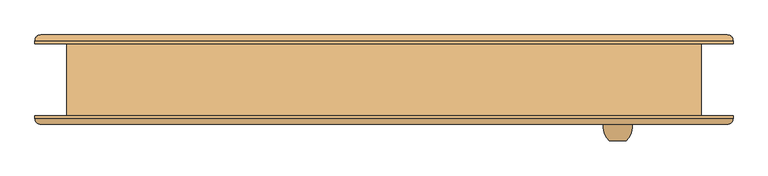
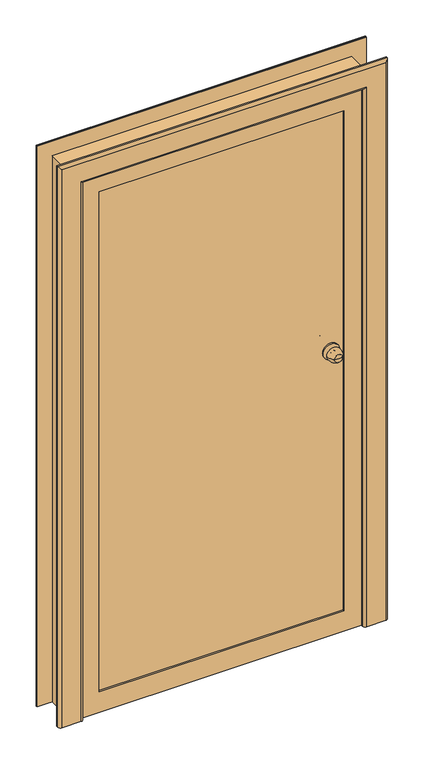
"""IFC4 building model written with IfcOpenShell, lengths in millimetres: door geometry, Наружная дверь 1-Навесная - Один проем наружу с порогом - 31173-2003 : ДСН КЛН  М1 УЗ 2100-1100 ГОСТ 31173-2003."""

from ifc_helpers import new_model, si_unit, point, frame, origin, place, context, project, spatial, polyline, circle_curve, ellipse_curve, trimmed, outline, extrude, faceted_brep, source, transform, mapped, element, save
from ifc_brep_helpers import plane_surface, cylinder_surface, revolved_surface, advanced_brep


def door_7e4ce2f0(model_context):
    return source(origin(), model_context, "Body", "SolidModel", [
        advanced_brep(
        [(390.0, -105.5, 1100.0), (405.0, -105.5, 1100.0), (420.0, -105.5, 1100.0), (430.0, -75.5, 1100.0), (380.0, -75.5, 1100.0), (423.0, -75.5, 1100.0), (387.0, -75.5, 1100.0), (415.0, -67.5, 1100.0), (395.0, -67.5, 1100.0), (415.0, -61.5, 1100.0), (395.0, -61.5, 1100.0), (435.0, -61.5, 1100.0), (375.0, -61.5, 1100.0), (435.0, -55.5, 1100.0), (375.0, -55.5, 1100.0)],
        [
            (0, 1),
            (1, 2),
            (2, 0, circle_curve(frame((405.0, -105.5, 1100.0), z_axis=(0.0, -1.0, 0.0), x_axis=(1.0, 0.0, 0.0)), 15.0)),
            (0, 2, circle_curve(frame((405.0, -105.5, 1100.0), z_axis=(0.0, -1.0, 0.0), x_axis=(1.0, 0.0, 0.0)), 15.0)),
            (2, 3, circle_curve(frame((395.3773735, -80.6257912, 1100.0), z_axis=(0.0, 0.0, 1.0), x_axis=(-1.0, 0.0, 0.0)), 35.0)),
            (3, 4, circle_curve(frame((405.0, -75.5, 1100.0), z_axis=(0.0, -1.0, 0.0), x_axis=(1.0, 0.0, 0.0)), 25.0)),
            (4, 0, circle_curve(frame((414.6226265, -80.6257912, 1100.0), z_axis=(0.0, 0.0, 1.0), x_axis=(1.0, 0.0, 0.0)), 35.0)),
            (4, 3, circle_curve(frame((405.0, -75.5, 1100.0), z_axis=(0.0, -1.0, 0.0), x_axis=(1.0, 0.0, 0.0)), 25.0)),
            (3, 5),
            (5, 6, circle_curve(frame((405.0, -75.5, 1100.0), z_axis=(0.0, -1.0, 0.0), x_axis=(1.0, 0.0, 0.0)), 18.0)),
            (6, 4),
            (6, 5, circle_curve(frame((405.0, -75.5, 1100.0), z_axis=(0.0, -1.0, 0.0), x_axis=(1.0, 0.0, 0.0)), 18.0)),
            (5, 7, circle_curve(frame((423.0, -67.5, 1100.0), z_axis=(0.0, 0.0, -1.0), x_axis=(-1.0, 0.0, 0.0)), 8.0)),
            (7, 8, circle_curve(frame((405.0, -67.5, 1100.0), z_axis=(0.0, -1.0, 0.0), x_axis=(1.0, 0.0, 0.0)), 10.0)),
            (8, 6, circle_curve(frame((387.0, -67.5, 1100.0), z_axis=(0.0, 0.0, -1.0), x_axis=(1.0, 0.0, 0.0)), 8.0)),
            (8, 7, circle_curve(frame((405.0, -67.5, 1100.0), z_axis=(0.0, -1.0, 0.0), x_axis=(1.0, 0.0, 0.0)), 10.0)),
            (7, 9),
            (9, 10, circle_curve(frame((405.0, -61.5, 1100.0), z_axis=(0.0, -1.0, 0.0), x_axis=(1.0, 0.0, 0.0)), 10.0)),
            (10, 8),
            (10, 9, circle_curve(frame((405.0, -61.5, 1100.0), z_axis=(0.0, -1.0, 0.0), x_axis=(1.0, 0.0, 0.0)), 10.0)),
            (11, 12, circle_curve(frame((405.0, -61.5, 1100.0), z_axis=(0.0, -1.0, 0.0), x_axis=(-1.0, 0.0, 0.0)), 30.0)),
            (12, 11, circle_curve(frame((405.0, -61.5, 1100.0), z_axis=(0.0, -1.0, 0.0), x_axis=(-1.0, 0.0, 0.0)), 30.0)),
            (13, 14, circle_curve(frame((405.0, -55.5, 1100.0), z_axis=(0.0, 1.0, 0.0), x_axis=(-1.0, 0.0, 0.0)), 30.0)),
            (14, 13, circle_curve(frame((405.0, -55.5, 1100.0), z_axis=(0.0, 1.0, 0.0), x_axis=(-1.0, 0.0, 0.0)), 30.0)),
            (12, 14),
            (13, 11),
        ],
        [
            plane_surface(frame((405.0, -105.5, 1100.0), z_axis=(0.0, -1.0, 0.0), x_axis=(1.0, 0.0, 0.0))),
            revolved_surface(trimmed(ellipse_curve(frame((395.3773735, -80.6257912, 1100.0), z_axis=(0.0, 0.0, 1.0), x_axis=(-1.0, 0.0, 0.0)), 35.0, 35.0), [point((420.0, -105.5, 1100.0))], [point((430.0, -75.5, 1100.0))], True, "CARTESIAN"), (405.0, -135.5, 1100.0), (0.0, 1.0, 0.0)),
            plane_surface(frame((405.0, -75.5, 1100.0), z_axis=(0.0, 1.0, 0.0), x_axis=(1.0, 0.0, 0.0))),
            revolved_surface(trimmed(ellipse_curve(frame((423.0, -67.5, 1100.0), z_axis=(0.0, 0.0, -1.0), x_axis=(-1.0, 0.0, 0.0)), 8.0, 8.0), [point((423.0, -75.5, 1100.0))], [point((415.0, -67.5, 1100.0))], True, "CARTESIAN"), (405.0, -135.5, 1100.0), (0.0, 1.0, 0.0)),
            cylinder_surface(frame((405.0, -135.5, 1100.0), z_axis=(0.0, 1.0, 0.0), x_axis=(1.0, 0.0, 0.0)), 10.0),
            plane_surface(frame((375.0, -61.5, 1100.0), z_axis=(0.0, -1.0, 0.0), x_axis=(0.0, 0.0, 1.0))),
            plane_surface(frame((375.0, -55.5, 1100.0), z_axis=(0.0, 1.0, 0.0), x_axis=(0.0, 0.0, -1.0))),
            cylinder_surface(frame((405.0, -55.5, 1100.0), z_axis=(0.0, -1.0, 0.0), x_axis=(-1.0, 0.0, 0.0)), 30.0),
        ],
        [
            (0, [[1, 2, 3]]),
            (0, [[-1, 4, -2]]),
            (1, [[5, 6, 7, -3]]),
            (1, [[-7, 8, -5, -4]]),
            (2, [[9, 10, 11, -6]]),
            (2, [[-11, 12, -9, -8]]),
            (3, [[13, 14, 15, -10]]),
            (3, [[-15, 16, -13, -12]]),
            (4, [[17, 18, 19, -14]]),
            (4, [[-19, 20, -17, -16]]),
            (5, [[21, 22], [-20, -18]]),
            (6, [[23, 24]]),
            (7, [[25, -23, 26, -22]]),
            (7, [[-26, -24, -25, -21]]),
        ],
    ),
        advanced_brep(
        [(420.0, 64.5, 1100.0), (405.0, 64.5, 1100.0), (390.0, 64.5, 1100.0), (380.0, 34.5, 1100.0), (430.0, 34.5, 1100.0), (387.0, 34.5, 1100.0), (423.0, 34.5, 1100.0), (395.0, 26.5, 1100.0), (415.0, 26.5, 1100.0), (395.0, 20.5, 1100.0), (415.0, 20.5, 1100.0), (375.0, 20.5, 1100.0), (435.0, 20.5, 1100.0), (375.0, 14.5, 1100.0), (435.0, 14.5, 1100.0)],
        [
            (0, 1),
            (1, 2),
            (2, 0, circle_curve(frame((405.0, 64.5, 1100.0), z_axis=(0.0, 1.0, 0.0), x_axis=(-1.0, 0.0, 0.0)), 15.0)),
            (0, 2, circle_curve(frame((405.0, 64.5, 1100.0), z_axis=(0.0, 1.0, 0.0), x_axis=(-1.0, 0.0, 0.0)), 15.0)),
            (2, 3, circle_curve(frame((414.6226265, 39.6257912, 1100.0), z_axis=(0.0, 0.0, 1.0), x_axis=(1.0, 0.0, 0.0)), 35.0)),
            (3, 4, circle_curve(frame((405.0, 34.5, 1100.0), z_axis=(0.0, 1.0, 0.0), x_axis=(-1.0, 0.0, 0.0)), 25.0)),
            (4, 0, circle_curve(frame((395.3773735, 39.6257912, 1100.0), z_axis=(0.0, 0.0, 1.0), x_axis=(-1.0, 0.0, 0.0)), 35.0)),
            (4, 3, circle_curve(frame((405.0, 34.5, 1100.0), z_axis=(0.0, 1.0, 0.0), x_axis=(-1.0, 0.0, 0.0)), 25.0)),
            (3, 5),
            (5, 6, circle_curve(frame((405.0, 34.5, 1100.0), z_axis=(0.0, 1.0, 0.0), x_axis=(-1.0, 0.0, 0.0)), 18.0)),
            (6, 4),
            (6, 5, circle_curve(frame((405.0, 34.5, 1100.0), z_axis=(0.0, 1.0, 0.0), x_axis=(-1.0, 0.0, 0.0)), 18.0)),
            (5, 7, circle_curve(frame((387.0, 26.5, 1100.0), z_axis=(0.0, 0.0, -1.0), x_axis=(1.0, 0.0, 0.0)), 8.0)),
            (7, 8, circle_curve(frame((405.0, 26.5, 1100.0), z_axis=(0.0, 1.0, 0.0), x_axis=(-1.0, 0.0, 0.0)), 10.0)),
            (8, 6, circle_curve(frame((423.0, 26.5, 1100.0), z_axis=(0.0, 0.0, -1.0), x_axis=(-1.0, 0.0, 0.0)), 8.0)),
            (8, 7, circle_curve(frame((405.0, 26.5, 1100.0), z_axis=(0.0, 1.0, 0.0), x_axis=(-1.0, 0.0, 0.0)), 10.0)),
            (7, 9),
            (9, 10, circle_curve(frame((405.0, 20.5, 1100.0), z_axis=(0.0, 1.0, 0.0), x_axis=(-1.0, 0.0, 0.0)), 10.0)),
            (10, 8),
            (10, 9, circle_curve(frame((405.0, 20.5, 1100.0), z_axis=(0.0, 1.0, 0.0), x_axis=(-1.0, 0.0, 0.0)), 10.0)),
            (11, 12, circle_curve(frame((405.0, 20.5, 1100.0), z_axis=(0.0, 1.0, 0.0), x_axis=(1.0, 0.0, 0.0)), 30.0)),
            (12, 11, circle_curve(frame((405.0, 20.5, 1100.0), z_axis=(0.0, 1.0, 0.0), x_axis=(1.0, 0.0, 0.0)), 30.0)),
            (13, 14, circle_curve(frame((405.0, 14.5, 1100.0), z_axis=(0.0, -1.0, 0.0), x_axis=(1.0, 0.0, 0.0)), 30.0)),
            (14, 13, circle_curve(frame((405.0, 14.5, 1100.0), z_axis=(0.0, -1.0, 0.0), x_axis=(1.0, 0.0, 0.0)), 30.0)),
            (12, 14),
            (13, 11),
        ],
        [
            plane_surface(frame((405.0, 64.5, 1100.0), z_axis=(0.0, 1.0, 0.0), x_axis=(-1.0, 0.0, 0.0))),
            revolved_surface(trimmed(ellipse_curve(frame((414.6226265, 39.6257912, 1100.0), z_axis=(0.0, 0.0, 1.0), x_axis=(1.0, 0.0, 0.0)), 35.0, 35.0), [point((390.0, 64.5, 1100.0))], [point((380.0, 34.5, 1100.0))], True, "CARTESIAN"), (405.0, 94.5, 1100.0), (0.0, -1.0, 0.0)),
            plane_surface(frame((405.0, 34.5, 1100.0), z_axis=(0.0, -1.0, 0.0), x_axis=(-1.0, 0.0, 0.0))),
            revolved_surface(trimmed(ellipse_curve(frame((387.0, 26.5, 1100.0), z_axis=(0.0, 0.0, -1.0), x_axis=(1.0, 0.0, 0.0)), 8.0, 8.0), [point((387.0, 34.5, 1100.0))], [point((395.0, 26.5, 1100.0))], True, "CARTESIAN"), (405.0, 94.5, 1100.0), (0.0, -1.0, 0.0)),
            cylinder_surface(frame((405.0, 94.5, 1100.0), z_axis=(0.0, -1.0, 0.0), x_axis=(-1.0, 0.0, 0.0)), 10.0),
            plane_surface(frame((435.0, 20.5, 1100.0), z_axis=(0.0, 1.0, 0.0), x_axis=(0.0, 0.0, 1.0))),
            plane_surface(frame((435.0, 14.5, 1100.0), z_axis=(0.0, -1.0, 0.0), x_axis=(0.0, 0.0, -1.0))),
            cylinder_surface(frame((405.0, 14.5, 1100.0), z_axis=(0.0, 1.0, 0.0), x_axis=(1.0, 0.0, 0.0)), 30.0),
        ],
        [
            (0, [[1, 2, 3]]),
            (0, [[-1, 4, -2]]),
            (1, [[5, 6, 7, -3]]),
            (1, [[-7, 8, -5, -4]]),
            (2, [[9, 10, 11, -6]]),
            (2, [[-11, 12, -9, -8]]),
            (3, [[13, 14, 15, -10]]),
            (3, [[-15, 16, -13, -12]]),
            (4, [[17, 18, 19, -14]]),
            (4, [[-19, 20, -17, -16]]),
            (5, [[21, 22], [-20, -18]]),
            (6, [[23, 24]]),
            (7, [[25, -23, 26, -22]]),
            (7, [[-26, -24, -25, -21]]),
        ],
    ),
        faceted_brep([(485.0, 14.5, 42.0), (485.0, 9.5, 42.0), (-485.0, 9.5, 42.0), (-485.0, 14.5, 42.0), (485.0, 14.5, 2055.0), (485.0, 9.5, 2055.0), (-485.0, 9.5, 2055.0), (465.0, 9.5, 2035.0), (465.0, 9.5, 62.0), (-465.0, 9.5, 62.0), (-465.0, 9.5, 2035.0), (-485.0, 14.5, 2055.0), (465.0, -55.5, 2035.0), (465.0, -55.5, 62.0), (-465.0, -55.5, 62.0), (-465.0, -55.5, 2035.0)], [[[0, 1, 2, 3]], [[4, 5, 1, 0]], [[5, 6, 2, 1], [7, 8, 9, 10]], [[2, 6, 11, 3]], [[11, 4, 0, 3]], [[7, 12, 13, 8]], [[9, 8, 13, 14]], [[15, 10, 9, 14]], [[12, 15, 14, 13]], [[4, 11, 6, 5]], [[7, 10, 15, 12]]]),
        extrude(outline(polyline([(0.0, 515.0), (0.0, 530.0), (2100.0, 530.0), (2100.0, -530.0), (0.0, -530.0), (0.0, -515.0), (2085.0, -515.0), (2085.0, 515.0), (0.0, 515.0)])), frame((0.0, 7.5, 0.0), z_axis=(0.0, 1.0, 0.0), x_axis=(0.0, 0.0, 1.0)), (0.0, 0.0, 1.0), 55.0),
        faceted_brep([(530.0, 7.5, 0.0), (530.0, -62.5, 0.0), (-530.0, -62.5, 0.0), (-530.0, 7.5, 0.0), (-530.0, -62.5, 2100.0), (-530.0, 7.5, 2100.0), (530.0, -62.5, 2100.0), (-450.0, -62.5, 2020.0), (450.0, -62.5, 2020.0), (450.0, -62.5, 80.0), (-450.0, -62.5, 80.0), (530.0, 7.5, 2100.0), (-470.0, 7.5, 60.0), (470.0, 7.5, 60.0), (470.0, 7.5, 2040.0), (-470.0, 7.5, 2040.0), (470.0, -57.5, 60.0), (-470.0, -57.5, 60.0), (-470.0, -57.5, 2040.0), (470.0, -57.5, 2040.0), (-450.0, -57.5, 80.0), (450.0, -57.5, 80.0), (450.0, -57.5, 2020.0), (-450.0, -57.5, 2020.0)], [[[0, 1, 2, 3]], [[3, 2, 4, 5]], [[2, 1, 6, 4], [7, 8, 9, 10]], [[5, 11, 0, 3], [12, 13, 14, 15]], [[16, 13, 12, 17]], [[17, 12, 15, 18]], [[18, 19, 16, 17], [20, 21, 22, 23]], [[9, 21, 20, 10]], [[10, 20, 23, 7]], [[11, 6, 1, 0]], [[19, 14, 13, 16]], [[8, 22, 21, 9]], [[5, 4, 6, 11]], [[18, 15, 14, 19]], [[7, 23, 22, 8]]]),
        advanced_brep(
        [(-605.0, -62.5, 0.0), (-515.0, -62.5, 0.0), (-515.0, -67.5, 0.0), (-525.0, -77.5, 0.0), (-595.0, -77.5, 0.0), (-605.0, -67.5, 0.0), (-605.0, -62.5, 2175.0), (605.0, -62.5, 2175.0), (605.0, -62.5, 0.0), (515.0, -62.5, 0.0), (515.0, -62.5, 2085.0), (-515.0, -62.5, 2085.0), (-515.0, -67.5, 2085.0), (-525.0, -77.5, 2095.0), (525.0, -77.5, 2095.0), (525.0, -77.5, 0.0), (595.0, -77.5, 0.0), (595.0, -77.5, 2165.0), (-595.0, -77.5, 2165.0), (-605.0, -67.5, 2175.0), (605.0, -67.5, 2175.0), (605.0, -67.5, 0.0), (515.0, -67.5, 0.0), (515.0, -67.5, 2085.0)],
        [
            (0, 1),
            (1, 2),
            (2, 3, circle_curve(frame((-525.0, -67.5, 0.0), z_axis=(0.0, 0.0, -1.0), x_axis=(-1.0, 0.0, 0.0)), 10.0)),
            (3, 4),
            (4, 5, circle_curve(frame((-595.0, -67.5, 0.0), z_axis=(0.0, 0.0, -1.0), x_axis=(-1.0, 0.0, 0.0)), 10.0)),
            (5, 0),
            (0, 6),
            (6, 7),
            (7, 8),
            (8, 9),
            (9, 10),
            (10, 11),
            (11, 1),
            (11, 12),
            (12, 2),
            (12, 13, ellipse_curve(frame((-525.0, -67.5, 2095.0), z_axis=(-0.7071067811865475, 0.0, -0.7071067811865475), x_axis=(0.7071067811865474, 0.0, -0.7071067811865476)), 14.1421356, 10.0)),
            (13, 3),
            (13, 14),
            (14, 15),
            (15, 16),
            (16, 17),
            (17, 18),
            (18, 4),
            (18, 19, ellipse_curve(frame((-595.0, -67.5, 2165.0), z_axis=(-0.7071067811865475, 0.0, -0.7071067811865475), x_axis=(0.7071067811865474, 0.0, -0.7071067811865476)), 14.1421356, 10.0)),
            (19, 5),
            (19, 6),
            (7, 20),
            (20, 21),
            (21, 8),
            (21, 16, circle_curve(frame((595.0, -67.5, 0.0), z_axis=(0.0, 0.0, -1.0), x_axis=(1.0, 0.0, 0.0)), 10.0)),
            (15, 22, circle_curve(frame((525.0, -67.5, 0.0), z_axis=(0.0, 0.0, -1.0), x_axis=(1.0, 0.0, 0.0)), 10.0)),
            (22, 9),
            (23, 10),
            (22, 23),
            (14, 23, ellipse_curve(frame((525.0, -67.5, 2095.0), z_axis=(0.7071067811865475, 0.0, -0.7071067811865475), x_axis=(0.7071067811865474, 0.0, 0.7071067811865476)), 14.1421356, 10.0)),
            (20, 17, ellipse_curve(frame((595.0, -67.5, 2165.0), z_axis=(0.7071067811865475, 0.0, -0.7071067811865475), x_axis=(0.7071067811865474, 0.0, 0.7071067811865476)), 14.1421356, 10.0)),
            (23, 12),
            (20, 19),
        ],
        [
            plane_surface(frame((-550.0, -62.5, 0.0), z_axis=(0.0, 0.0, -1.0), x_axis=(0.0, -1.0, 0.0))),
            plane_surface(frame((-605.0, -62.5, 0.0), z_axis=(0.0, 1.0, 0.0), x_axis=(0.0, 0.0, 1.0))),
            plane_surface(frame((-515.0, -62.5, 0.0), z_axis=(1.0, 0.0, 0.0), x_axis=(0.0, 0.0, 1.0))),
            cylinder_surface(frame((-525.0, -67.5, 0.0), z_axis=(0.0, 0.0, -1.0), x_axis=(-1.0, 0.0, 0.0)), 10.0),
            plane_surface(frame((-525.0, -77.5, 0.0), z_axis=(0.0, -1.0, 0.0), x_axis=(0.0, 0.0, 1.0))),
            cylinder_surface(frame((-595.0, -67.5, 0.0), z_axis=(0.0, 0.0, -1.0), x_axis=(-1.0, 0.0, 0.0)), 10.0),
            plane_surface(frame((-605.0, -67.5, 0.0), z_axis=(-1.0, 0.0, 0.0), x_axis=(0.0, 0.0, 1.0))),
            plane_surface(frame((605.0, -67.5, 2175.0), z_axis=(1.0, 0.0, 0.0), x_axis=(0.0, 0.0, -1.0))),
            plane_surface(frame((550.0, -62.5, 0.0), z_axis=(0.0, 0.0, -1.0), x_axis=(0.0, -1.0, 0.0))),
            plane_surface(frame((515.0, -62.5, 2085.0), z_axis=(-1.0, 0.0, 0.0), x_axis=(0.0, 0.0, -1.0))),
            cylinder_surface(frame((525.0, -67.5, 2120.0), z_axis=(0.0, 0.0, 1.0), x_axis=(1.0, 0.0, 0.0)), 10.0),
            cylinder_surface(frame((595.0, -67.5, 2120.0), z_axis=(0.0, 0.0, 1.0), x_axis=(1.0, 0.0, 0.0)), 10.0),
            plane_surface(frame((-515.0, -62.5, 2085.0), z_axis=(0.0, 0.0, -1.0), x_axis=(1.0, 0.0, 0.0))),
            cylinder_surface(frame((-550.0, -67.5, 2095.0), z_axis=(-1.0, 0.0, 0.0), x_axis=(0.0, 0.0, 1.0)), 10.0),
            cylinder_surface(frame((-550.0, -67.5, 2165.0), z_axis=(-1.0, 0.0, 0.0), x_axis=(0.0, 0.0, 1.0)), 10.0),
            plane_surface(frame((-605.0, -67.5, 2175.0), z_axis=(0.0, 0.0, 1.0), x_axis=(1.0, 0.0, 0.0))),
        ],
        [
            (0, [[1, 2, 3, 4, 5, 6]]),
            (1, [[-1, 7, 8, 9, 10, 11, 12, 13]]),
            (2, [[-2, -13, 14, 15]]),
            (3, [[-3, -15, 16, 17]]),
            (4, [[-4, -17, 18, 19, 20, 21, 22, 23]]),
            (5, [[-5, -23, 24, 25]]),
            (6, [[-6, -25, 26, -7]]),
            (7, [[27, 28, 29, -9]]),
            (8, [[-29, 30, -20, 31, 32, -10]]),
            (9, [[33, -11, -32, 34]]),
            (10, [[35, -34, -31, -19]]),
            (11, [[36, -21, -30, -28]]),
            (12, [[-14, -12, -33, 37]]),
            (13, [[-16, -37, -35, -18]]),
            (14, [[-24, -22, -36, 38]]),
            (15, [[-26, -38, -27, -8]]),
        ],
    ),
        advanced_brep(
        [(605.0, 62.5, 0.0), (515.0, 62.5, 0.0), (515.0, 67.5, 0.0), (525.0, 77.5, 0.0), (595.0, 77.5, 0.0), (605.0, 67.5, 0.0), (605.0, 62.5, 2175.0), (-605.0, 62.5, 2175.0), (-605.0, 62.5, 0.0), (-515.0, 62.5, 0.0), (-515.0, 62.5, 2085.0), (515.0, 62.5, 2085.0), (515.0, 67.5, 2085.0), (525.0, 77.5, 2095.0), (-525.0, 77.5, 2095.0), (-525.0, 77.5, 0.0), (-595.0, 77.5, 0.0), (-595.0, 77.5, 2165.0), (595.0, 77.5, 2165.0), (605.0, 67.5, 2175.0), (-605.0, 67.5, 2175.0), (-605.0, 67.5, 0.0), (-515.0, 67.5, 0.0), (-515.0, 67.5, 2085.0)],
        [
            (0, 1),
            (1, 2),
            (2, 3, circle_curve(frame((525.0, 67.5, 0.0), z_axis=(0.0, 0.0, -1.0), x_axis=(1.0, 0.0, 0.0)), 10.0)),
            (3, 4),
            (4, 5, circle_curve(frame((595.0, 67.5, 0.0), z_axis=(0.0, 0.0, -1.0), x_axis=(1.0, 0.0, 0.0)), 10.0)),
            (5, 0),
            (0, 6),
            (6, 7),
            (7, 8),
            (8, 9),
            (9, 10),
            (10, 11),
            (11, 1),
            (11, 12),
            (12, 2),
            (12, 13, ellipse_curve(frame((525.0, 67.5, 2095.0), z_axis=(0.7071067811865475, 0.0, -0.7071067811865475), x_axis=(-0.7071067811865474, 0.0, -0.7071067811865476)), 14.1421356, 10.0)),
            (13, 3),
            (13, 14),
            (14, 15),
            (15, 16),
            (16, 17),
            (17, 18),
            (18, 4),
            (18, 19, ellipse_curve(frame((595.0, 67.5, 2165.0), z_axis=(0.7071067811865475, 0.0, -0.7071067811865475), x_axis=(-0.7071067811865474, 0.0, -0.7071067811865476)), 14.1421356, 10.0)),
            (19, 5),
            (19, 6),
            (7, 20),
            (20, 21),
            (21, 8),
            (21, 16, circle_curve(frame((-595.0, 67.5, 0.0), z_axis=(0.0, 0.0, -1.0), x_axis=(-1.0, 0.0, 0.0)), 10.0)),
            (15, 22, circle_curve(frame((-525.0, 67.5, 0.0), z_axis=(0.0, 0.0, -1.0), x_axis=(-1.0, 0.0, 0.0)), 10.0)),
            (22, 9),
            (23, 10),
            (22, 23),
            (14, 23, ellipse_curve(frame((-525.0, 67.5, 2095.0), z_axis=(-0.7071067811865475, 0.0, -0.7071067811865475), x_axis=(-0.7071067811865474, 0.0, 0.7071067811865476)), 14.1421356, 10.0)),
            (20, 17, ellipse_curve(frame((-595.0, 67.5, 2165.0), z_axis=(-0.7071067811865475, 0.0, -0.7071067811865475), x_axis=(-0.7071067811865474, 0.0, 0.7071067811865476)), 14.1421356, 10.0)),
            (23, 12),
            (20, 19),
        ],
        [
            plane_surface(frame((550.0, 62.5, 0.0), z_axis=(0.0, 0.0, -1.0), x_axis=(0.0, -1.0, 0.0))),
            plane_surface(frame((605.0, 62.5, 0.0), z_axis=(0.0, -1.0, 0.0), x_axis=(0.0, 0.0, 1.0))),
            plane_surface(frame((515.0, 62.5, 0.0), z_axis=(-1.0, 0.0, 0.0), x_axis=(0.0, 0.0, 1.0))),
            cylinder_surface(frame((525.0, 67.5, 0.0), z_axis=(0.0, 0.0, -1.0), x_axis=(1.0, 0.0, 0.0)), 10.0),
            plane_surface(frame((525.0, 77.5, 0.0), z_axis=(0.0, 1.0, 0.0), x_axis=(0.0, 0.0, 1.0))),
            cylinder_surface(frame((595.0, 67.5, 0.0), z_axis=(0.0, 0.0, -1.0), x_axis=(1.0, 0.0, 0.0)), 10.0),
            plane_surface(frame((605.0, 67.5, 0.0), z_axis=(1.0, 0.0, 0.0), x_axis=(0.0, 0.0, 1.0))),
            plane_surface(frame((-605.0, 67.5, 2175.0), z_axis=(-1.0, 0.0, 0.0), x_axis=(0.0, 0.0, -1.0))),
            plane_surface(frame((-550.0, 62.5, 0.0), z_axis=(0.0, 0.0, -1.0), x_axis=(0.0, -1.0, 0.0))),
            plane_surface(frame((-515.0, 62.5, 2085.0), z_axis=(1.0, 0.0, 0.0), x_axis=(0.0, 0.0, -1.0))),
            cylinder_surface(frame((-525.0, 67.5, 2120.0), z_axis=(0.0, 0.0, 1.0), x_axis=(-1.0, 0.0, 0.0)), 10.0),
            cylinder_surface(frame((-595.0, 67.5, 2120.0), z_axis=(0.0, 0.0, 1.0), x_axis=(-1.0, 0.0, 0.0)), 10.0),
            plane_surface(frame((515.0, 62.5, 2085.0), z_axis=(0.0, 0.0, -1.0), x_axis=(-1.0, 0.0, 0.0))),
            cylinder_surface(frame((550.0, 67.5, 2095.0), z_axis=(1.0, 0.0, 0.0), x_axis=(0.0, 0.0, 1.0)), 10.0),
            cylinder_surface(frame((550.0, 67.5, 2165.0), z_axis=(1.0, 0.0, 0.0), x_axis=(0.0, 0.0, 1.0)), 10.0),
            plane_surface(frame((605.0, 67.5, 2175.0), z_axis=(0.0, 0.0, 1.0), x_axis=(-1.0, 0.0, 0.0))),
        ],
        [
            (0, [[1, 2, 3, 4, 5, 6]]),
            (1, [[-1, 7, 8, 9, 10, 11, 12, 13]]),
            (2, [[-2, -13, 14, 15]]),
            (3, [[-3, -15, 16, 17]]),
            (4, [[-4, -17, 18, 19, 20, 21, 22, 23]]),
            (5, [[-5, -23, 24, 25]]),
            (6, [[-6, -25, 26, -7]]),
            (7, [[27, 28, 29, -9]]),
            (8, [[-29, 30, -20, 31, 32, -10]]),
            (9, [[33, -11, -32, 34]]),
            (10, [[35, -34, -31, -19]]),
            (11, [[36, -21, -30, -28]]),
            (12, [[-14, -12, -33, 37]]),
            (13, [[-16, -37, -35, -18]]),
            (14, [[-24, -22, -36, 38]]),
            (15, [[-26, -38, -27, -8]]),
        ],
    ),
        extrude(outline(polyline([(0.0, 530.0), (0.0, 550.0), (2120.0, 550.0), (2120.0, -550.0), (0.0, -550.0), (0.0, -530.0), (2100.0, -530.0), (2100.0, 530.0), (0.0, 530.0)])), frame((0.0, -62.5, 0.0), z_axis=(0.0, 1.0, 0.0), x_axis=(0.0, 0.0, 1.0)), (0.0, 0.0, 1.0), 125.0),
    ])


if __name__ == "__main__":
    model = new_model("IFC4")
    model_context = context("Model", 3, world=origin())
    ifc_project = project(units=[si_unit("LENGTHUNIT", "METRE", prefix="MILLI")], contexts=[model_context])
    site = spatial("IfcSite", under=ifc_project)
    building = spatial("IfcBuilding", under=site)
    placement = place(None, origin())
    door_shape = door_7e4ce2f0(model_context)
    element("IfcDoor", 1, ObjectType="Наружная дверь 1-Навесная - Один проем наружу с порогом - 31173-2003 : ДСН КЛН  М1 УЗ 2100-1100 ГОСТ 31173-2003", at=placement, inside=building, context=model_context, shape_type="MappedRepresentation", body=[
        mapped(door_shape, transform((0.0, 0.0, 0.0), x_axis=(1.0, 0.0, 0.0), y_axis=(0.0, 1.0, 0.0), z_axis=(0.0, 0.0, 1.0))),
    ])
    save(model, "model.ifc")

# Revit data of these elements
# Type "Наружная дверь 1-Навесная - Один проем наружу с порогом - 31173-2003 : ДСН КЛН  М1 УЗ 2100-1100 ГОСТ 31173-2003"
#   Type Mark = "152"
#   Description = "ДСН КЛН  М1 УЗ 2100-900 ГОСТ 31173-2003"
#   Проекционное соединение по ширине = 90 mm
#   Rough Width = 1100 mm
#   Rough Height = 2120 mm
#   Угол проема [instance default] = 30°
#   Толщина_Тепл_Изоляции = 20 mm
#   Heat Transfer Coefficient (U) = 3.7021 W/(m²·K)
#   Height = 2100 mm
#   Width = 1060 mm
#   Ширина каркаса = 60 mm
#   Толщина каркаса = 70 mm
#   Вставка двери [instance default] = 0 mm
#   Правая сторона = no
#   Левая сторона = yes
#   Function = 1
#   Обрезка = Сталь
#   Панель = Сталь
#   Тепловая изоляция = Тепловая изоляция
#   Кадр = Сталь
#   Дверная ручка = Металл
#   Visual Light Transmittance = 0
#   Solar Heat Gain Coefficient = 0
#   Construction Type Id = ""
#   Wall Closure = (empty or 0)
#   Analytic Construction = (empty or 0)
# Element 1 (IfcDoor, "Наружная дверь 1-Навесная - Один проем наружу с порогом - 31173-2003 : ДСН КЛН  М1 УЗ 2100-1100 ГОСТ 31173-2003")
#   Materials on its faces: "Сталь", "Металл", "Тепловая изоляция"
# Materials
#   "Сталь": class "Металл", colour RGB 247 247 247, transparency 0
#   "Тепловая изоляция": class "Пластмасса", colour RGB 185 154 119, transparency 0, Cost = 0
#   "Металл": class "Металл", colour RGB 249 249 249, transparency 0
